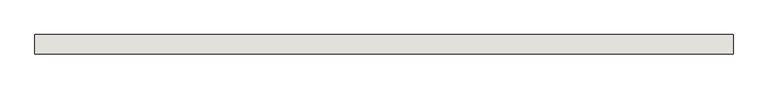
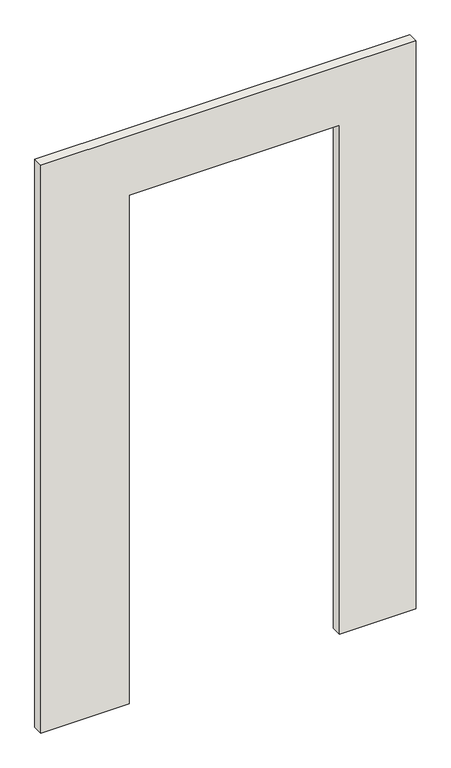
"""IFC4 building model written with IfcOpenShell, lengths in millimetres: wall geometry, 0_3d."""

from ifc_helpers import new_model, si_unit, frame, origin, place, context, project, spatial, polyline, outline, extrude, source, transform, mapped, element, save


def wall_94fef32f(model_context):
    return source(origin(), model_context, "Body", "SweptSolid", [
        extrude(outline(polyline([(2580.0, 1434.0747536), (0.0, 1434.0747536), (0.0, 1800.0), (2880.0, 1800.0), (2880.0, 0.0), (0.0, 0.0), (0.0, 424.0747536), (2580.0, 424.0747536), (2580.0, 1434.0747536)])), frame((0.0, 0.0, 0.0), z_axis=(0.0, 1.0, 0.0), x_axis=(0.0, 0.0, 1.0)), (0.0, 0.0, 1.0), 50.0),
    ])


if __name__ == "__main__":
    model = new_model("IFC4")
    model_context = context("Model", 3, world=origin())
    ifc_project = project(units=[si_unit("LENGTHUNIT", "METRE", prefix="MILLI")], contexts=[model_context])
    site = spatial("IfcSite", under=ifc_project)
    building = spatial("IfcBuilding", under=site)
    placement = place(None, origin())
    wall_shape = wall_94fef32f(model_context)
    element("IfcWall", 1, ObjectType="0_3d", at=placement, inside=building, context=model_context, shape_type="MappedRepresentation", body=[
        mapped(wall_shape, transform((0.0, 0.0, 0.0), x_axis=(1.0, 0.0, 0.0), y_axis=(0.0, 1.0, 0.0), z_axis=(0.0, 0.0, 1.0))),
    ])
    save(model, "model.ifc")

# Revit data of these elements
# Element 1 (IfcWall, "0_3d")
#   Materials on its faces: "glas"
# Materials
#   "glas": class "Unassigned", colour RGB 250 253 254, transparency 0.95
